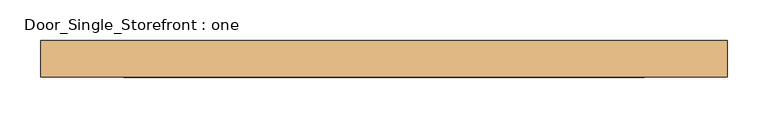
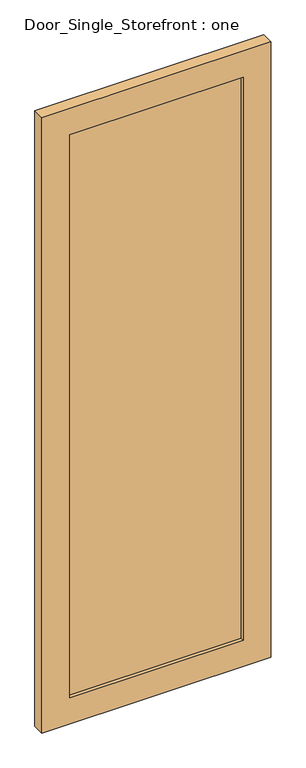
"""IFC4 building model written with IfcOpenShell, lengths in millimetres: door geometry, Door_Single_Storefront : one."""

from ifc_helpers import new_model, si_unit, frame, origin, place, context, project, spatial, polyline, outline, extrude, source, transform, mapped, element, save


def door_single_storefront_one_3caf9fd9(model_context):
    return source(origin(), model_context, "Body", "SweptSolid", [
        extrude(outline(polyline([(2387.6, -419.89375), (0.0, -419.89375), (0.0, 419.89375), (2387.6, 419.89375), (2387.6, -419.89375)]), holes=[polyline([(101.6, 318.29375), (101.6, -318.29375), (2286.0, -318.29375), (2286.0, 318.29375), (101.6, 318.29375)])]), frame((0.0, -25.4, 0.0), z_axis=(0.0, 1.0, 0.0), x_axis=(0.0, 0.0, 1.0)), (0.0, 0.0, 1.0), 44.45),
        extrude(outline(polyline([(318.29375, 6.35), (318.29375, -12.7), (-318.29375, -12.7), (-318.29375, 6.35), (318.29375, 6.35)])), frame((0.0, 0.0, 101.6), z_axis=(0.0, 0.0, 1.0), x_axis=(1.0, 0.0, 0.0)), (0.0, 0.0, 1.0), 2184.4),
    ])


if __name__ == "__main__":
    model = new_model("IFC4")
    model_context = context("Model", 3, world=origin())
    ifc_project = project(units=[si_unit("LENGTHUNIT", "METRE", prefix="MILLI")], contexts=[model_context])
    site = spatial("IfcSite", under=ifc_project)
    building = spatial("IfcBuilding", under=site)
    placement = place(None, origin())
    door_single_storefront_one_shape = door_single_storefront_one_3caf9fd9(model_context)
    element("IfcDoor", 1, ObjectType="Door_Single_Storefront : one", at=placement, inside=building, context=model_context, shape_type="MappedRepresentation", body=[
        mapped(door_single_storefront_one_shape, transform((0.0, 0.0, 0.0), x_axis=(1.0, 0.0, 0.0), y_axis=(0.0, 1.0, 0.0), z_axis=(0.0, 0.0, 1.0))),
    ])
    save(model, "model.ifc")

# Revit data of these elements
# Type "Door_Single_Storefront : one"
#   Type Mark = "27"
#   Analytic Construction = "<None>"
#   Stile_Width = 0' - 4"
#   Door_Thickness = 0' - 1 3/4"
#   Door_Offset = 0' - 1"
#   Glass_Material = Glass
#   Frame_Material = Aluminum
#   Function = (empty or 0)
# Element 1 (IfcDoor, "Door_Single_Storefront : one")
#   Materials on its faces: "Aluminum", "Glass"
# Materials
#   "Glass": class "Glass", colour RGB 142 168 196, transparency 0.75, Description = "Soda Lime Glass", Cost = 0
#   "Aluminum": class "Metal", colour RGB 226 226 226, transparency 0, Description = "Aluminum 6061", Cost = 0
